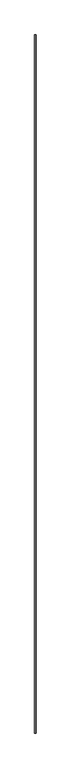
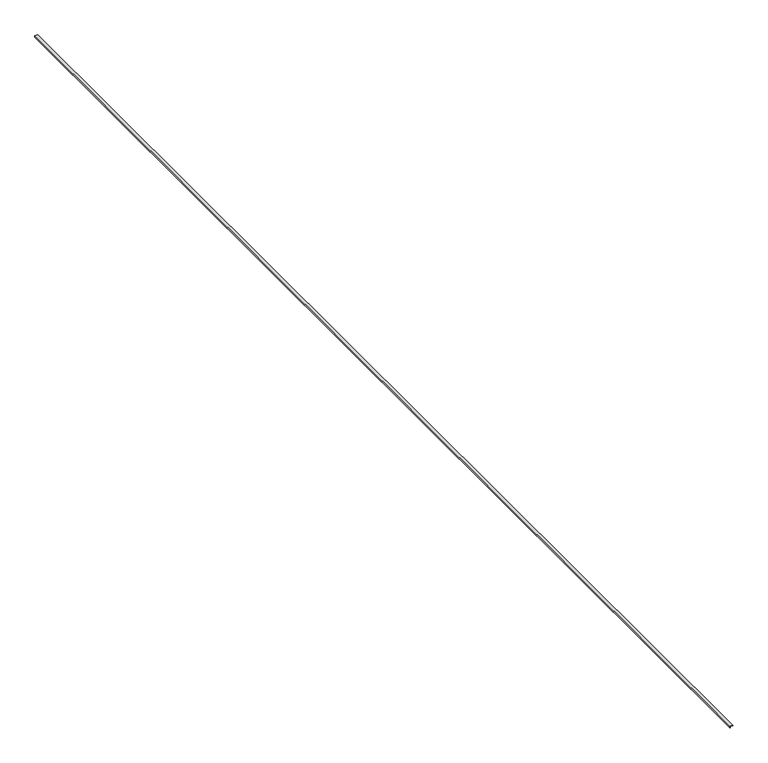
"""IFC4 building model written with IfcOpenShell, lengths in millimetres: proxy geometry, Generic Models 7:Generic Models 1:8:Generic Models 1:8 : Generic Models 7:Generic Models 1:337419:7 : Generic Models 7:Generic Models 1:8:Generic Models 1:8 : Generic Models 7:Generic Models 1:337419:315935."""

import ifcopenshell
import ifcopenshell.guid

model = None  # the IFC model being written
_history = None  # IfcOwnerHistory: only IFC2X3 demands one
_inside = {}  # id of a spatial element -> (the spatial element, [elements in it])
_under = {}  # id of a project, library or spatial element -> (it, [spatial elements below it])
_declared = {}  # id of a project -> (the project, [libraries it declares])
_typed = {}  # id of a type object -> (the type object, [elements of that type])
_made_of = {}  # id of a material, layer set ... -> (it, [elements and type objects made of it])


def new_model(schema):
    """Start an empty IFC model of exactly this schema.

    Asked for "IFC4X3", IfcOpenShell would pick the latest addendum, in which some entities
    have other attributes; the version numbers below select the first issue.
    IFC2X3 requires an IfcOwnerHistory on every rooted entity: one is made here for all.
    """
    global model, _history
    if schema == "IFC4X3":
        model = ifcopenshell.file(schema_version=(4, 3, 0, 0))
    else:
        model = ifcopenshell.file(schema=schema)
    _inside.clear()
    _under.clear()
    _declared.clear()
    _typed.clear()
    _made_of.clear()
    _history = None
    if model.schema == "IFC2X3":
        org = make("IfcOrganization", Name="unknown")
        user = make(
            "IfcPersonAndOrganization",
            ThePerson=make("IfcPerson", FamilyName="unknown"),
            TheOrganization=org,
        )
        app = make(
            "IfcApplication",
            ApplicationDeveloper=org,
            Version="unknown",
            ApplicationFullName="unknown",
            ApplicationIdentifier="unknown",
        )
        _history = make(
            "IfcOwnerHistory",
            OwningUser=user,
            OwningApplication=app,
            ChangeAction="ADDED",
            CreationDate=0,
        )
    return model


def make(cls, **values):
    """One entity of the class cls with the attributes given. An attribute that is None is left unset."""
    return model.create_entity(
        cls, **{name: value for name, value in values.items() if value is not None}
    )


def rooted(cls, **values):
    """An entity with a GlobalId (a new one), such as an element, a storey or a relation."""
    return make(cls, GlobalId=ifcopenshell.guid.new(), OwnerHistory=_history, **values)


def si_unit(unit_type, name, prefix=None):
    """IfcSIUnit, for example si_unit("LENGTHUNIT", "METRE", prefix="MILLI")."""
    return make("IfcSIUnit", UnitType=unit_type, Prefix=prefix, Name=name)


def assignment(units):
    """IfcUnitAssignment: the units of a project."""
    return None if units is None else make("IfcUnitAssignment", Units=units)


def point(xyz):
    """IfcCartesianPoint."""
    return None if xyz is None else make("IfcCartesianPoint", Coordinates=xyz)


def direction(xyz):
    """IfcDirection."""
    return None if xyz is None else make("IfcDirection", DirectionRatios=xyz)


def frame(location, z_axis=None, x_axis=None):
    """IfcAxis2Placement3D, a coordinate frame: its origin and axes. An axis left out is left unset."""
    return make(
        "IfcAxis2Placement3D",
        Location=point(location),
        Axis=direction(z_axis),
        RefDirection=direction(x_axis),
    )


def origin():
    """The frame at (0, 0, 0) with its axes left unset."""
    return frame((0.0, 0.0, 0.0))


def place(relative_to, where):
    """IfcLocalPlacement: puts the frame where relative to a parent placement (None: the world)."""
    return make(
        "IfcLocalPlacement", PlacementRelTo=relative_to, RelativePlacement=where
    )


def context(
    kind, dimensions, precision=None, world=None, true_north=None, identifier=None
):
    """IfcGeometricRepresentationContext, for example the 3D "Model" context."""
    return make(
        "IfcGeometricRepresentationContext",
        ContextIdentifier=identifier,
        ContextType=kind,
        CoordinateSpaceDimension=dimensions,
        Precision=precision,
        WorldCoordinateSystem=world,
        TrueNorth=true_north,
    )


def project(units=None, contexts=None):
    """IfcProject with its units and contexts."""
    return rooted(
        "IfcProject",
        Name="project",
        RepresentationContexts=contexts,
        UnitsInContext=assignment(units),
    )


def spatial(cls, under=None, at=None, **own):
    """A site, building, storey or space (cls), placed at a placement, below another one or the project."""
    s = rooted(cls, ObjectPlacement=at, **own)
    if under is not None:
        _under.setdefault(under.id(), (under, []))[1].append(s)
    return s


def polyline(points):
    """IfcPolyline through the points."""
    return make("IfcPolyline", Points=[point(p) for p in points])


def outline(outer, holes=None, kind="AREA"):
    """IfcArbitraryClosedProfileDef: a profile drawn as a closed curve; with holes, ...WithVoids."""
    if holes is None:
        return make("IfcArbitraryClosedProfileDef", ProfileType=kind, OuterCurve=outer)
    return make(
        "IfcArbitraryProfileDefWithVoids",
        ProfileType=kind,
        OuterCurve=outer,
        InnerCurves=holes,
    )


def extrude(swept, where, along, depth):
    """IfcExtrudedAreaSolid: the profile swept, set in the frame where, extruded along a direction by depth."""
    return make(
        "IfcExtrudedAreaSolid",
        SweptArea=swept,
        Position=where,
        ExtrudedDirection=direction(along),
        Depth=depth,
    )


def shape(context_of_items, identifier, shape_type, items):
    """IfcShapeRepresentation: the items that make up one representation, for example the "Body"."""
    return make(
        "IfcShapeRepresentation",
        ContextOfItems=context_of_items,
        RepresentationIdentifier=identifier,
        RepresentationType=shape_type,
        Items=items,
    )


def source(mapping_origin, context_of_items, identifier, shape_type, items):
    """IfcRepresentationMap: a shape defined once, which mapped items show again and again."""
    return make(
        "IfcRepresentationMap",
        MappingOrigin=mapping_origin,
        MappedRepresentation=shape(context_of_items, identifier, shape_type, items),
    )


def transform(
    local_origin,
    x_axis=None,
    y_axis=None,
    z_axis=None,
    scale=None,
    scale2=None,
    scale3=None,
    uniform=True,
):
    """IfcCartesianTransformationOperator3D, or its non-uniform kind. x_axis, y_axis, z_axis: its Axis1, 2, 3."""
    if uniform:
        return make(
            "IfcCartesianTransformationOperator3D",
            Axis1=direction(x_axis),
            Axis2=direction(y_axis),
            LocalOrigin=point(local_origin),
            Scale=scale,
            Axis3=direction(z_axis),
        )
    return make(
        "IfcCartesianTransformationOperator3DnonUniform",
        Axis1=direction(x_axis),
        Axis2=direction(y_axis),
        LocalOrigin=point(local_origin),
        Scale=scale,
        Axis3=direction(z_axis),
        Scale2=scale2,
        Scale3=scale3,
    )


def mapped(mapping_source, mapping_target):
    """IfcMappedItem: shows the shape of a source again, moved by a transform."""
    return make(
        "IfcMappedItem", MappingSource=mapping_source, MappingTarget=mapping_target
    )


def made_of(thing, what):
    """Note that an element or type object is made of a material, layer set ...; save() writes the relation."""
    if what is not None:
        _made_of.setdefault(what.id(), (what, []))[1].append(thing)
    return thing


def element(
    cls,
    number,
    at=None,
    inside=None,
    cuts=None,
    type_object=None,
    material=None,
    context=None,
    identifier="Body",
    shape_type=None,
    held_by="IfcProductDefinitionShape",
    body=None,
    shapes=None,
    **own,
):
    """One element of the class cls, such as IfcWall. Its Tag is "e" and its number.

    at: its placement. inside: the storey or other place that contains it. cuts: it is an
    opening in that element (IfcRelVoidsElement). A single representation is given by context,
    identifier, shape_type and body (its items); several are given by shapes. held_by: the class
    of the entity that holds the representations. save() writes the other relations.
    """
    e = rooted(cls, Tag="e%d" % number, ObjectPlacement=at, **own)
    if body is not None:
        shapes = [shape(context, identifier, shape_type, body)]
    if shapes is not None:
        e.Representation = make(held_by, Representations=shapes)
    if inside is not None:
        _inside.setdefault(inside.id(), (inside, []))[1].append(e)
    if cuts is not None:
        rooted(
            "IfcRelVoidsElement", RelatingBuildingElement=cuts, RelatedOpeningElement=e
        )
    if type_object is not None:
        _typed.setdefault(type_object.id(), (type_object, []))[1].append(e)
    return made_of(e, material)


def aggregate(whole, parts):
    """IfcRelAggregates: a whole, such as a stair, and the parts it consists of."""
    return rooted("IfcRelAggregates", RelatingObject=whole, RelatedObjects=parts)


def save(model, path):
    """Write the relations noted so far, then the file.

    IfcRelAggregates (storeys below a building ...), IfcRelContainedInSpatialStructure (elements
    in a storey), IfcRelDefinesByType, IfcRelAssociatesMaterial and IfcRelDeclares: one each for
    every whole, place, type object, material and project.
    """
    for whole, parts in _under.values():
        aggregate(whole, parts)
    for where, things in _inside.values():
        rooted(
            "IfcRelContainedInSpatialStructure",
            RelatedElements=things,
            RelatingStructure=where,
        )
    for kind, things in _typed.values():
        rooted("IfcRelDefinesByType", RelatedObjects=things, RelatingType=kind)
    for what, things in _made_of.values():
        rooted("IfcRelAssociatesMaterial", RelatedObjects=things, RelatingMaterial=what)
    for by, libraries in _declared.values():
        rooted("IfcRelDeclares", RelatingContext=by, RelatedDefinitions=libraries)
    model.write(path)


def generic_models_8cadb35e(model_context):
    return source(origin(), model_context, "Body", "SweptSolid", [
        extrude(outline(polyline([(3671.5071615, 560245.7438791), (3712.5900973, 560245.7438791), (3715.6565635, 560319.3390665), (3719.1638003, 560319.1929316), (3715.9571615, 560242.2335991), (3671.5071615, 560242.2335991), (3671.5071615, 560245.7438791)])), frame((0.0, -578670.4913841, 0.0), z_axis=(0.0, 1.0, 0.0), x_axis=(0.0, 0.0, 1.0)), (0.0, 0.0, 1.0), 35486.9749999),
    ])


if __name__ == "__main__":
    model = new_model("IFC4")
    model_context = context("Model", 3, world=origin())
    ifc_project = project(units=[si_unit("LENGTHUNIT", "METRE", prefix="MILLI")], contexts=[model_context])
    site = spatial("IfcSite", under=ifc_project)
    building = spatial("IfcBuilding", under=site)
    placement = place(None, origin())
    generic_models_shape = generic_models_8cadb35e(model_context)
    element("IfcBuildingElementProxy", 1, Name="Generic Models 7:Generic Models 1:8:Generic Models 1:8 : Generic Models 7:Generic Models 1:337419:7 : Generic Models 7:Generic Models 1:8:Generic Models 1:8 : Generic Models 7:Generic Models 1:337419:315935", ObjectType="Generic Models 7:Generic Models 1:8:Generic Models 1:8 : Generic Models 7:Generic Models 1:337419:7 : Generic Models 7:Generic Models 1:8:Generic Models 1:8 : Generic Models 7:Generic Models 1:337419:315935", at=placement, inside=building, context=model_context, shape_type="MappedRepresentation", body=[
        mapped(generic_models_shape, transform((0.0, 0.0, 0.0), x_axis=(1.0, 0.0, 0.0), y_axis=(0.0, 1.0, 0.0), z_axis=(0.0, 0.0, 1.0))),
    ])
    save(model, "model.ifc")

# Revit data of these elements
# Type "Generic Models 7:Generic Models 1:8:Generic Models 1:8 : Generic Models 7:Generic Models 1:337419:7 : Generic Models 7:Generic Models 1:8:Generic Models 1:8 : Generic Models 7:Generic Models 1:337419:315935"
#   NameOverride = "Generic Models 7:Generic Models 1:8:Generic Models 1:8 : Generic Models 7:Generic Models 1:337419:315935"
#   ObjectTypeOverride = "Generic Models 1:8 : Generic Models 7:Generic Models 1:337419"
#   Reference = "Generic Models 1"
#   Tag = "315935"
# Element 1 (IfcBuildingElementProxy, "Generic Models 7:Generic Models 1:8:Generic Models 1:8 : Generic Models 7:Generic Models 1:337419:7 : Generic Models 7:Generic Models 1:8:Generic Models 1:8 : Generic Models 7:Generic Models 1:337419:315935")
#   Materials on its faces: "11 GA. ALUM. BRAKE METAL"
# Materials
#   "11 GA. ALUM. BRAKE METAL": class "Unassigned", colour RGB 210 209 208, transparency 0, Cost = 0
